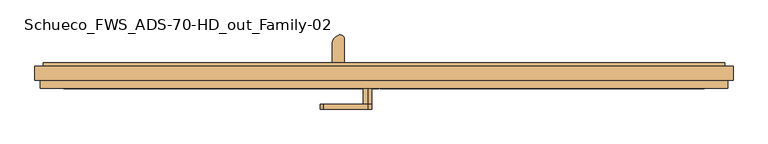
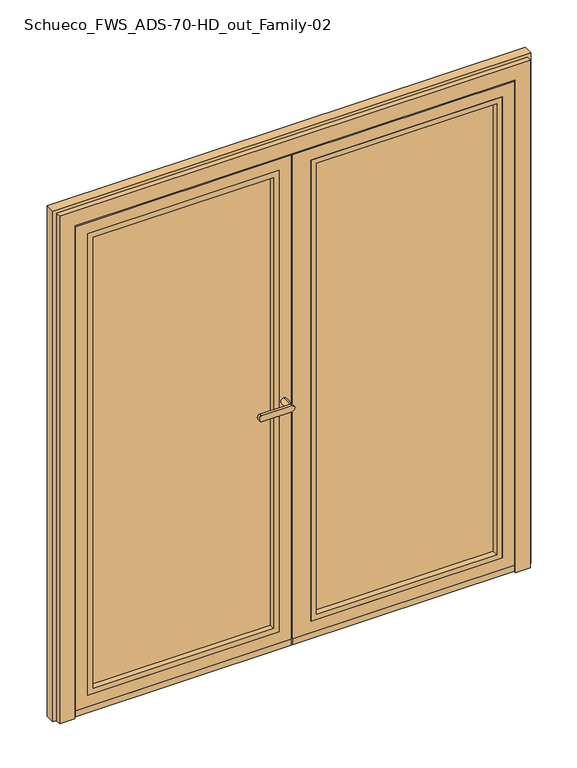
"""IFC4 building model written with IfcOpenShell, lengths in millimetres: door geometry, Schueco_FWS_ADS-70-HD_out_Family-02 : FWS SI insert unit."""

from ifc_helpers import new_model, si_unit, point, frame, frame_2d, origin, place, context, project, spatial, polyline, circle_curve, ellipse_curve, trimmed, segment, composite_curve, outline, extrude, faceted_brep, source, transform, mapped, element, save
from ifc_brep_helpers import plane_surface, cylinder_surface, extruded_surface, advanced_brep


def schueco_fws_ads_70_hd_out_family_02_d351c64d(model_context):
    return source(origin(), model_context, "Body", "SolidModel", [
        faceted_brep([(875.0, -52.4997281, 33.0), (875.0, -52.4997281, 2075.0), (875.0, -61.0000038, 2075.0), (875.0, -61.0000038, 33.0), (-10.0, -61.0000038, 33.0), (-10.0, -52.4997281, 33.0), (5.0, -52.4997281, 33.0), (885.0, -52.4997281, 23.0), (885.0, -52.4997281, 2085.0), (5.0, -52.4997281, 2085.0), (5.0, -52.4997281, 2075.0), (5.0, -52.4997281, 23.0), (-10.0, -61.0000038, 2075.0), (63.0, -61.0000038, 81.0), (63.0, -61.0000038, 2027.0), (827.0, -61.0000038, 2027.0), (827.0, -61.0000038, 81.0), (827.0, 0.5000388, 2027.0), (827.0, 0.5000388, 81.0), (63.0, 0.5000388, 81.0), (63.0, 0.5000388, 2027.0), (88.0, 0.5000388, 106.0), (88.0, 0.5000388, 2002.0), (802.0, 0.5000388, 2002.0), (802.0, 0.5000388, 106.0), (802.0, 8.9999962, 2002.0), (802.0, 8.9999962, 106.0), (88.0, 8.9999962, 106.0), (88.0, 8.9999962, 2002.0), (900.0, 8.9999962, 8.0), (15.0, 8.9999962, 8.0), (15.0, 8.9999962, 2100.0), (900.0, 8.9999962, 2100.0), (900.0, 0.5000388, 2100.0), (900.0, 0.5000388, 8.0), (15.0, 0.5000388, 8.0), (15.0, 0.5000388, 2100.0), (15.0, 0.5000388, 2085.0), (885.0, 0.5000388, 2085.0), (885.0, 0.5000388, 23.0), (15.0, 0.5000388, 23.0), (5.0, 0.5000388, 23.0), (5.0, 0.5000388, 2085.0), (-10.0, -52.4997281, 2075.0)], [[[0, 1, 2, 3]], [[3, 4, 5, 6, 0]], [[7, 8, 9, 10, 1, 0, 6, 11]], [[2, 12, 4, 3], [13, 14, 15, 16]], [[16, 15, 17, 18]], [[18, 19, 13, 16]], [[19, 20, 14, 13]], [[18, 17, 20, 19], [21, 22, 23, 24]], [[24, 23, 25, 26]], [[26, 27, 21, 24]], [[27, 28, 22, 21]], [[29, 30, 31, 32], [26, 25, 28, 27]], [[29, 32, 33, 34]], [[34, 35, 30, 29]], [[33, 36, 37, 38, 39, 40, 35, 34]], [[39, 38, 8, 7]], [[7, 11, 41, 40, 39]], [[11, 6, 10, 9, 42, 41]], [[1, 10, 43, 12, 2]], [[20, 17, 15, 14]], [[28, 25, 23, 22]], [[32, 31, 36, 33]], [[9, 8, 38, 37, 42]], [[43, 10, 6, 5]], [[4, 12, 43, 5]], [[37, 36, 31, 30, 35, 40]], [[40, 41, 42, 37]]]),
        extrude(outline(polyline([(81.0, 63.0), (81.0, 827.0), (2027.0, 827.0), (2027.0, 63.0), (81.0, 63.0)]), holes=[polyline([(103.0, 805.0), (103.0, 85.0), (2005.0, 85.0), (2005.0, 805.0), (103.0, 805.0)])]), frame((0.0, -61.0000038, 0.0), z_axis=(0.0, 1.0, 0.0), x_axis=(0.0, 0.0, 1.0)), (0.0, 0.0, 1.0), 23.5000426),
        extrude(outline(polyline([(63.0, -37.4999612), (63.0, 0.5000388), (827.0, 0.5000388), (827.0, -37.4999612), (63.0, -37.4999612)])), frame((0.0, 0.0, 81.0), z_axis=(0.0, 0.0, 1.0), x_axis=(1.0, 0.0, 0.0)), (0.0, 0.0, 1.0), 1946.0),
        extrude(outline(composite_curve([segment(polyline([(-26.243662, 23.0), (-26.243662, 4.2956275)]), True, "CONTINUOUS"), segment(trimmed(circle_curve(frame_2d((-36.8960283, 15.355415)), 15.3555139), [point((-26.243662, 4.2956275))], [point((-47.5483946, 4.2956275))], False, "CARTESIAN"), True, "CONTINUOUS"), segment(polyline([(-47.5483946, 4.2956275), (-47.5483946, 23.0), (-26.243662, 23.0)]), True, "CONTINUOUS")], self_intersect=False)), frame((5.0, 0.0, 0.0), z_axis=(1.0, 0.0, 0.0), x_axis=(0.0, 1.0, 0.0)), (0.0, 0.0, 1.0), 880.0),
        extrude(outline(polyline([(875.0, -61.0000038), (-10.0, -61.0000038), (-10.0, -52.4997281), (875.0, -52.4997281), (875.0, -61.0000038)])), frame((0.0, 0.0, 8.0), z_axis=(0.0, 0.0, 1.0), x_axis=(1.0, 0.0, 0.0)), (0.0, 0.0, 1.0), 25.0),
        extrude(outline(composite_curve([segment(polyline([(-141.6673236, 8.9997177), (-141.6673236, 59.1618682)]), True, "CONTINUOUS"), segment(trimmed(circle_curve(frame_2d((-114.4889059, 59.1618682)), 27.1784177), [point((-141.6673236, 59.1618682))], [point((-124.0260015, 84.6120194))], False, "CARTESIAN"), True, "CONTINUOUS"), segment(trimmed(circle_curve(frame_2d((-119.9485005, 73.7310321)), 11.6198924), [point((-124.0260015, 84.6120194))], [point((-108.3286081, 73.7310321))], False, "CARTESIAN"), True, "CONTINUOUS"), segment(polyline([(-108.3286081, 73.7310321), (-108.3286081, 8.9997177), (-141.6673236, 8.9997177)]), True, "CONTINUOUS")], self_intersect=False)), frame((0.0, 0.0, 2043.9340013), z_axis=(0.0, 0.0, 1.0), x_axis=(1.0, 0.0, 0.0)), (0.0, 0.0, 1.0), 4.0),
        extrude(outline(polyline([(-141.6673236, 12.9997177), (-108.3286081, 12.9997177), (-108.3286081, 8.9997177), (-141.6673236, 8.9997177), (-141.6673236, 12.9997177)])), frame((0.0, 0.0, 2013.9340013), z_axis=(0.0, 0.0, 1.0), x_axis=(1.0, 0.0, 0.0)), (0.0, 0.0, 1.0), 30.0),
        extrude(outline(polyline([(-141.6673236, 12.9997177), (-108.3286081, 12.9997177), (-108.3286081, 8.9997177), (-141.6673236, 8.9997177), (-141.6673236, 12.9997177)])), frame((0.0, 0.0, 56.9340013), z_axis=(0.0, 0.0, 1.0), x_axis=(1.0, 0.0, 0.0)), (0.0, 0.0, 1.0), 30.0),
        extrude(outline(composite_curve([segment(polyline([(-141.6673236, 8.9997177), (-141.6673236, 59.1618682)]), True, "CONTINUOUS"), segment(trimmed(circle_curve(frame_2d((-114.4889059, 59.1618682)), 27.1784177), [point((-141.6673236, 59.1618682))], [point((-124.0260015, 84.6120194))], False, "CARTESIAN"), True, "CONTINUOUS"), segment(trimmed(circle_curve(frame_2d((-119.9485005, 73.7310321)), 11.6198924), [point((-124.0260015, 84.6120194))], [point((-108.3286081, 73.7310321))], False, "CARTESIAN"), True, "CONTINUOUS"), segment(polyline([(-108.3286081, 73.7310321), (-108.3286081, 8.9997177), (-141.6673236, 8.9997177)]), True, "CONTINUOUS")], self_intersect=False)), frame((0.0, 0.0, 52.9340013), z_axis=(0.0, 0.0, 1.0), x_axis=(1.0, 0.0, 0.0)), (0.0, 0.0, 1.0), 4.0),
        advanced_brep(
        [(-112.282924, 57.5977179, 2043.9340013), (-137.717076, 72.2821425, 2043.9340013), (-112.282924, 57.5977179, 56.9340013), (-137.717076, 72.2821425, 56.9340013)],
        [
            (0, 1, ellipse_curve(frame((-125.0, 64.9399302, 2043.9340013), z_axis=(0.0, 0.0, 1.0000000000000002), x_axis=(0.5000002582658958, 0.866025254674503, 0.0)), 21.5840887, 14.6844171)),
            (1, 0, ellipse_curve(frame((-125.0, 64.9399302, 2043.9340013), z_axis=(0.0, 0.0, 1.0000000000000002), x_axis=(0.5000002582658958, 0.866025254674503, 0.0)), 21.5840887, 14.6844171)),
            (2, 3, ellipse_curve(frame((-125.0, 64.9399302, 56.9340013), z_axis=(0.0, 0.0, -1.0000000000000002), x_axis=(-0.866025254674503, 0.5000002582658958, 0.0)), 14.6844171, 21.5840887)),
            (3, 2, ellipse_curve(frame((-125.0, 64.9399302, 56.9340013), z_axis=(0.0, 0.0, -1.0000000000000002), x_axis=(-0.866025254674503, 0.5000002582658958, 0.0)), 14.6844171, 21.5840887)),
            (0, 2),
            (3, 1),
        ],
        [
            plane_surface(frame((-137.717076, 72.2821425, 2043.9340013), z_axis=(0.0, 0.0, 1.0000000000000002), x_axis=(0.5000002582658958, 0.866025254674503, 0.0))),
            plane_surface(frame((-137.717076, 72.2821425, 56.9340013), z_axis=(0.0, 0.0, -1.0000000000000002), x_axis=(-0.5000002582658958, -0.866025254674503, 0.0))),
            extruded_surface(trimmed(ellipse_curve(frame((-125.0, 64.9399302, 56.9340013), z_axis=(0.0, 0.0, -1.0000000000000002), x_axis=(-0.866025254674503, 0.5000002582658958, 0.0)), 14.6844171, 21.5840887), [point((-137.717076, 72.2821425, 56.9340013))], [point((-112.282924, 57.5977179, 56.9340013))], True, "CARTESIAN"), (0.0, 0.0, -1987.0), 1987.0),
            extruded_surface(trimmed(ellipse_curve(frame((-125.0, 64.9399302, 56.9340013), z_axis=(0.0, 0.0, -1.0000000000000002), x_axis=(-0.866025254674503, 0.5000002582658958, 0.0)), 14.6844171, 21.5840887), [point((-112.282924, 57.5977179, 56.9340013))], [point((-137.717076, 72.2821425, 56.9340013))], True, "CARTESIAN"), (0.0, 0.0, -1987.0), 1987.0),
        ],
        [
            (0, [[1, 2]]),
            (1, [[3, 4]]),
            (2, [[5, -4, 6, -1]]),
            (3, [[-6, -3, -5, -2]]),
        ],
    ),
        advanced_brep(
        [(-45.0, -117.0002518, 1038.0113692), (-45.0, -117.0002518, 1061.9886308), (-166.6617926, -117.0002518, 1061.9886308), (-166.6617926, -117.0002518, 1038.0113692), (-45.0, -104.5001648, 1061.9886308), (-45.0, -104.5001648, 1038.0113692), (-166.6617926, -104.5001648, 1038.0113692), (-166.6617926, -104.5001648, 1061.9886308), (-45.0, -61.0002823, 1038.0113692), (-45.0, -61.0002823, 1061.9886308)],
        [
            (0, 1, circle_curve(frame((-45.0, -117.0002518, 1050.0), z_axis=(0.0, -1.0, 0.0), x_axis=(0.0, 0.0, 1.0)), 11.9886308)),
            (1, 2),
            (2, 3, ellipse_curve(frame((-166.6617926, -117.0002518, 1050.0), z_axis=(0.0, -1.0, 0.0), x_axis=(0.0, 0.0, -1.0)), 11.9886308, 7.9050795)),
            (3, 0),
            (4, 5, circle_curve(frame((-45.0, -104.5001648, 1050.0), z_axis=(0.0, -1.0, 0.0), x_axis=(0.0, 0.0, 1.0)), 11.9886308)),
            (5, 6),
            (6, 7, ellipse_curve(frame((-166.6617926, -104.5001648, 1050.0), z_axis=(0.0, 1.0, 0.0), x_axis=(0.0, 0.0, -1.0)), 11.9886308, 7.9050795)),
            (7, 4),
            (3, 6),
            (5, 0),
            (2, 7),
            (1, 4),
            (5, 4, circle_curve(frame((-45.0, -104.5001648, 1050.0), z_axis=(0.0, -1.0, 0.0), x_axis=(0.0, 0.0, 1.0)), 11.9886308)),
            (8, 9, circle_curve(frame((-45.0, -61.0002823, 1050.0), z_axis=(0.0, 1.0, 0.0), x_axis=(0.0, 0.0, 1.0)), 11.9886308)),
            (9, 8, circle_curve(frame((-45.0, -61.0002823, 1050.0), z_axis=(0.0, 1.0, 0.0), x_axis=(0.0, 0.0, 1.0)), 11.9886308)),
            (8, 5),
            (4, 9),
        ],
        [
            plane_surface(frame((-166.6617926, -117.0002518, 1038.0113692), z_axis=(0.0, -1.0, 0.0), x_axis=(-1.0, 0.0, 0.0))),
            plane_surface(frame((-166.6617926, -104.5001648, 1038.0113692), z_axis=(0.0, 1.0, 0.0), x_axis=(1.0, 0.0, 0.0))),
            plane_surface(frame((-45.0, -117.0002518, 1038.0113692), z_axis=(0.0, 0.0, -1.0), x_axis=(0.0, 1.0, 0.0))),
            extruded_surface(trimmed(ellipse_curve(frame((-166.6617926, -104.5001648, 1050.0), z_axis=(0.0, 1.0, 0.0), x_axis=(0.0, 0.0, -1.0)), 11.9886308, 7.9050795), [point((-166.6617926, -104.5001648, 1038.0113692))], [point((-166.6617926, -104.5001648, 1061.9886308))], True, "CARTESIAN"), (0.0, 12.500086999999994, 0.0), 12.500086999999994),
            plane_surface(frame((-166.6617926, -117.0002518, 1061.9886308), z_axis=(0.0, 0.0, 1.0), x_axis=(0.0, 1.0, 0.0))),
            cylinder_surface(frame((-45.0, -104.5001648, 1050.0), z_axis=(0.0, -1.0, 0.0), x_axis=(0.0, 0.0, 1.0)), 11.9886308),
            plane_surface(frame((-45.0, -61.0002823, 1061.9886308), z_axis=(0.0, 1.0, 0.0), x_axis=(-1.0, 0.0, 0.0))),
            cylinder_surface(frame((-45.0, -61.0002823, 1050.0), z_axis=(0.0, -1.0, 0.0), x_axis=(0.0, 0.0, 1.0)), 11.9886308),
        ],
        [
            (0, [[1, 2, 3, 4]]),
            (1, [[5, 6, 7, 8]]),
            (2, [[9, -6, 10, -4]]),
            (3, [[11, -7, -9, -3]]),
            (4, [[12, -8, -11, -2]]),
            (5, [[-10, 13, -12, -1]]),
            (6, [[14, 15]]),
            (7, [[16, -5, 17, -14]]),
            (7, [[-17, -13, -16, -15]]),
        ],
    ),
        faceted_brep([(-875.0, -52.5000065, 33.0), (-875.0, -61.0002823, 33.0), (-875.0, -61.0002823, 2075.0), (-875.0, -52.5000065, 2075.0), (-17.0, -52.5000065, 33.0), (-15.0, -52.5000065, 33.0), (-15.0, -61.0002823, 33.0), (-17.0, -61.0002823, 33.0), (-885.0, -52.5000065, 23.0), (-5.0, -52.5000065, 23.0), (-5.0, -52.5000065, 2085.0), (-885.0, -52.5000065, 2085.0), (-15.0, -52.5000065, 2075.0), (-17.0, -52.5000065, 2075.0), (-15.0, -61.0002823, 2075.0), (-17.0, -61.0002823, 2075.0), (-63.0, -61.0002823, 81.0), (-827.0, -61.0002823, 81.0), (-827.0, -61.0002823, 2027.0), (-63.0, -61.0002823, 2027.0), (-827.0, 0.4997603, 81.0), (-827.0, 0.4997603, 2027.0), (-63.0, 0.4997603, 81.0), (-63.0, 0.4997603, 2027.0), (-88.0, 0.4997603, 106.0), (-802.0, 0.4997603, 106.0), (-802.0, 0.4997603, 2002.0), (-88.0, 0.4997603, 2002.0), (-802.0, 8.9997177, 106.0), (-802.0, 8.9997177, 2002.0), (-88.0, 8.9997177, 106.0), (-88.0, 8.9997177, 2002.0), (10.0, 8.9997177, 8.0), (-900.0, 8.9997177, 8.0), (-900.0, 8.9997177, 2100.0), (10.0, 8.9997177, 2100.0), (-900.0, 0.4997603, 8.0), (-900.0, 0.4997603, 2100.0), (10.0, 0.4997603, 8.0), (10.0, 0.4997603, 2100.0), (-5.0, 0.4997603, 23.0), (-885.0, 0.4997603, 23.0), (-885.0, 0.4997603, 2085.0), (-5.0, 0.4997603, 2085.0)], [[[0, 1, 2, 3]], [[1, 0, 4, 5, 6, 7]], [[8, 9, 10, 11], [12, 5, 4, 0, 3, 13]], [[6, 5, 12, 14]], [[6, 14, 15, 2, 1, 7], [16, 17, 18, 19]], [[17, 20, 21, 18]], [[20, 17, 16, 22]], [[22, 16, 19, 23]], [[20, 22, 23, 21], [24, 25, 26, 27]], [[25, 28, 29, 26]], [[28, 25, 24, 30]], [[30, 24, 27, 31]], [[32, 33, 34, 35], [28, 30, 31, 29]], [[33, 36, 37, 34]], [[36, 33, 32, 38]], [[38, 32, 35, 39]], [[36, 38, 39, 37], [40, 41, 42, 43]], [[41, 8, 11, 42]], [[8, 41, 40, 9]], [[9, 40, 43, 10]], [[14, 12, 13, 3, 2, 15]], [[23, 19, 18, 21]], [[31, 27, 26, 29]], [[39, 35, 34, 37]], [[10, 43, 42, 11]]]),
        extrude(outline(polyline([(81.0, -63.0), (2027.0, -63.0), (2027.0, -827.0), (81.0, -827.0), (81.0, -63.0)]), holes=[polyline([(103.0, -805.0), (2005.0, -805.0), (2005.0, -85.0), (103.0, -85.0), (103.0, -805.0)])]), frame((0.0, -61.0002823, 0.0), z_axis=(0.0, 1.0, 0.0), x_axis=(0.0, 0.0, 1.0)), (0.0, 0.0, 1.0), 23.5000426),
        extrude(outline(polyline([(-63.0, -37.5002397), (-827.0, -37.5002397), (-827.0, 0.4997603), (-63.0, 0.4997603), (-63.0, -37.5002397)])), frame((0.0, 0.0, 81.0), z_axis=(0.0, 0.0, 1.0), x_axis=(1.0, 0.0, 0.0)), (0.0, 0.0, 1.0), 1946.0),
        extrude(outline(composite_curve([segment(polyline([(-26.2439405, 23.0), (-26.2439405, 4.2956275)]), True, "CONTINUOUS"), segment(trimmed(circle_curve(frame_2d((-36.8963068, 15.355415)), 15.3555139), [point((-26.2439405, 4.2956275))], [point((-47.548673, 4.2956275))], False, "CARTESIAN"), True, "CONTINUOUS"), segment(polyline([(-47.548673, 4.2956275), (-47.548673, 23.0), (-26.2439405, 23.0)]), True, "CONTINUOUS")], self_intersect=False)), frame((-885.0, 0.0, 0.0), z_axis=(1.0, 0.0, 0.0), x_axis=(0.0, 1.0, 0.0)), (0.0, 0.0, 1.0), 880.0),
        extrude(outline(polyline([(-875.0, -61.0002823), (-875.0, -52.5000065), (-15.0, -52.5000065), (-15.0, -61.0002823), (-875.0, -61.0002823)])), frame((0.0, 0.0, 8.0), z_axis=(0.0, 0.0, 1.0), x_axis=(1.0, 0.0, 0.0)), (0.0, 0.0, 1.0), 25.0),
        faceted_brep([(930.999943, 8.9997177, 2130.999943), (930.999943, 0.0, 2130.999943), (930.999943, 0.0, 0.0), (930.999943, 8.9997177, 0.0), (-954.0, 0.0, 0.0), (-954.0, 0.0, 2154.0), (954.0, 0.0, 2154.0), (954.0, 0.0, 0.0), (-930.999943, 0.0, 2130.999943), (-930.999943, 0.0, 0.0), (954.0, -38.0, 0.0), (940.0, -38.0, 0.0), (940.0, -61.0002823, 0.0), (880.0652914, -61.0002823, 0.0), (880.0652914, -52.5000065, 0.0), (893.4999114, -52.5000065, 0.0), (893.4999114, 0.4997603, 0.0), (904.9999827, 0.4997603, 0.0), (904.9999827, 8.9997177, 0.0), (-904.9999827, 8.9997177, 0.0), (-930.999943, 8.9997177, 0.0), (-930.999943, 8.9997177, 2130.999943), (904.9999827, 8.9997177, 2104.9999827), (-904.9999827, 8.9997177, 2104.9999827), (880.0652914, -61.0002823, 2080.0652914), (880.0652914, -52.5000065, 2080.0652914), (-880.0652914, -52.5000065, 0.0), (-893.4999114, -52.5000065, 0.0), (-893.4999114, -52.5000065, 2093.4999114), (893.4999114, -52.5000065, 2093.4999114), (-880.0652914, -52.5000065, 2080.0652914), (-940.0, -61.0002823, 0.0), (-880.0652914, -61.0002823, 0.0), (-880.0652914, -61.0002823, 2080.0652914), (940.0, -61.0002823, 2140.0), (-940.0, -61.0002823, 2140.0), (940.0, -38.0, 2140.0), (-954.0, -38.0, 0.0), (-940.0, -38.0, 0.0), (-940.0, -38.0, 2140.0), (954.0, -38.0, 2154.0), (-954.0, -38.0, 2154.0), (-904.9999827, 0.4997603, 0.0), (-893.4999114, 0.4997603, 0.0), (904.9999827, 0.4997603, 2104.9999827), (-904.9999827, 0.4997603, 2104.9999827), (893.4999114, 0.4997603, 2093.4999114), (-893.4999114, 0.4997603, 2093.4999114)], [[[0, 1, 2, 3]], [[4, 5, 6, 7, 2, 1, 8, 9]], [[3, 2, 7, 10, 11, 12, 13, 14, 15, 16, 17, 18]], [[19, 20, 21, 0, 3, 18, 22, 23]], [[24, 25, 14, 13]], [[26, 27, 28, 29, 15, 14, 25, 30]], [[31, 32, 33, 24, 13, 12, 34, 35]], [[34, 12, 11, 36]], [[37, 38, 39, 36, 11, 10, 40, 41]], [[4, 9, 20, 19, 42, 43, 27, 26, 32, 31, 38, 37]], [[20, 9, 8, 21]], [[18, 17, 44, 22]], [[42, 19, 23, 45]], [[32, 26, 30, 33]], [[31, 35, 39, 38]], [[4, 37, 41, 5]], [[6, 40, 10, 7]], [[43, 42, 45, 44, 17, 16, 46, 47]], [[16, 15, 29, 46]], [[27, 43, 47, 28]], [[21, 8, 1, 0]], [[33, 30, 25, 24]], [[35, 34, 36, 39]], [[23, 22, 44, 45]], [[5, 41, 40, 6]], [[47, 46, 29, 28]]]),
    ])


if __name__ == "__main__":
    model = new_model("IFC4")
    model_context = context("Model", 3, world=origin())
    ifc_project = project(units=[si_unit("LENGTHUNIT", "METRE", prefix="MILLI")], contexts=[model_context])
    site = spatial("IfcSite", under=ifc_project)
    building = spatial("IfcBuilding", under=site)
    placement = place(None, origin())
    schueco_fws_ads_70_hd_out_family_02_shape = schueco_fws_ads_70_hd_out_family_02_d351c64d(model_context)
    element("IfcDoor", 1, ObjectType="Schueco_FWS_ADS-70-HD_out_Family-02 : FWS SI insert unit", at=placement, inside=building, context=model_context, shape_type="MappedRepresentation", body=[
        mapped(schueco_fws_ads_70_hd_out_family_02_shape, transform((0.0, 0.0, 0.0), x_axis=(1.0, 0.0, 0.0), y_axis=(0.0, 1.0, 0.0), z_axis=(0.0, 0.0, 1.0))),
    ])
    save(model, "model.ifc")

# Revit data of these elements
# Type "Schueco_FWS_ADS-70-HD_out_Family-02 : FWS SI insert unit"
#   Type Mark = "46"
#   __NOTE__ = "Data describes the optimum values of the entire system. The properites of a selected design option have to be determined on an individual basis!"
#   Wind load resistance = "Class 2"
#   Watertightness = "Class 5A"
#   Thermal insulation = "Uf = 1.6 W/(m²K)"
#   Sound insulation = "to Rw 43 dB"
#   Schueco thermal insulation standard = "Thermally insulated"
#   Opening type = "Outward-opening, Flush-fitted"
#   Model = "Schueco ADS 70 HD"
#   Mechanical loading = "Class 2"
#   Maximum leaf width in mm = "1400"
#   Maximum leaf weight in kg = "200"
#   Maximum leaf height in mm = "3000"
#   Material = "Aluminium"
#   Long term functionality = "Class 6"
#   Construction Type = "Door, double-leaf, outward-opening"
#   Manufacturer = "Schueco International KG"
#   Glazing data = "Triple glazing 38mm"
#   Façade insert unit = "yes"
#   Family creation date = "08.2017"
#   Description = "Schueco Aluminium Door System (ADS)"
#   Burglar resistance = "Class RC 3"
#   Areas of use = "Public buildings"
#   Analytic Construction = "<None>"
#   Air permeability = "Class 2"
#   Width [instance default] = 997.455 mm
#   Leaf opening angle [instance default] = 0.00°
#   IOf_T = 38 mm
#   Height [instance default] = 2054.517 mm
#   Glazing area [instance default] = 1.20269 m²
#   F2_W [instance default] = 498.728 mm
#   F1_W [instance default] = 498.728 mm
#   Distance from bottom to handles [instance default] = 1050 mm
#   Clear opening width [instance default] = 849.455 mm
#   Active leaf width = 1100 mm
#   Standard threshold = no
#   Low level threshold = yes
#   Handles = yes
#   FWS SI insert unit = yes
#   FWS HI insert unit = no
#   All fields of identical width = yes
#   Glass = none
#   Frame = Alu
#   Fittings = none
# Element 1 (IfcDoor, "Schueco_FWS_ADS-70-HD_out_Family-02 : FWS SI insert unit")
#   Width = 1908 mm
#   Height = 2154 mm
#   Glazing area = 2.99568 m²
#   F2_W = 954 mm
#   F1_W = 954 mm
#   Clear opening width = 1760 mm
#   Materials on its faces: "Alu", "Glass"
# Materials
#   "Alu": class "Glas", colour RGB 140 140 140, transparency 0
#   "Glass": class "Glass", colour RGB 128 128 255, transparency 0.75, Description = "Soda Lime Glass", Cost = 0
